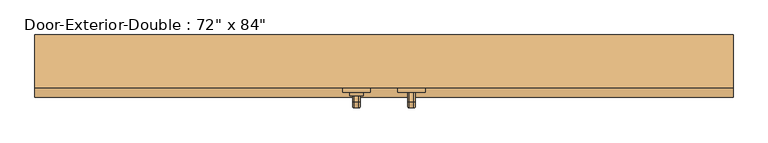
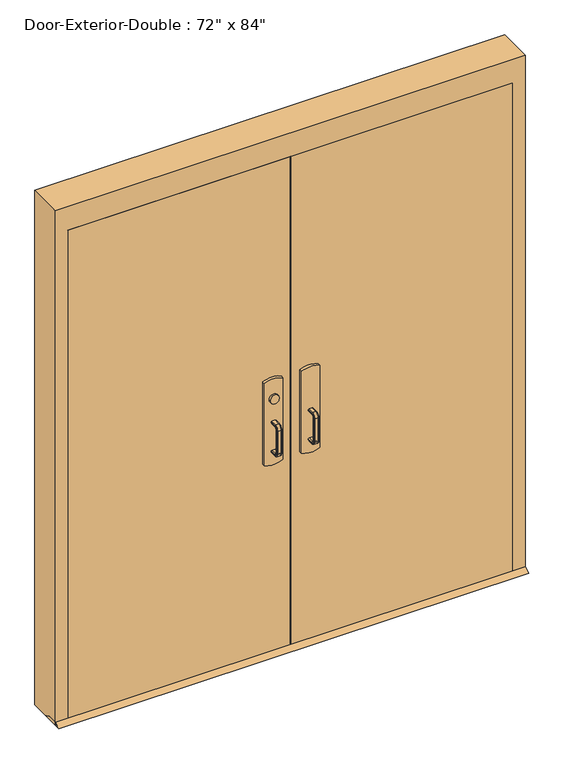
"""IFC4 building model written with IfcOpenShell, lengths in millimetres: door geometry."""

from ifc_helpers import new_model, si_unit, point, frame, frame_2d, origin, place, context, project, spatial, polyline, circle_curve, ellipse_curve, trimmed, segment, composite_curve, outline, extrude, faceted_brep, source, transform, mapped, element, save
from ifc_brep_helpers import plane_surface, cylinder_surface, revolved_surface, advanced_brep


def door_02051829(model_context):
    return source(origin(), model_context, "Body", "SolidModel", [
        extrude(outline(polyline([(-575.7333333, 0.0), (-76.2, 0.0), (-76.2, -6.35), (-575.7333333, -6.35), (-575.7333333, 0.0)])), frame((0.0, 0.0, 990.6), z_axis=(0.0, 0.0, 1.0), x_axis=(1.0, 0.0, 0.0)), (0.0, 0.0, 1.0), 50.8),
        advanced_brep(
        [(-12.7, -6.35, 1041.4), (-12.7, -6.35, 990.6), (-76.2, -6.35, 990.6), (-825.5, -6.35, 990.6), (-825.5, -6.35, 1041.4), (-76.2, -6.35, 1041.4), (-825.5, -38.1, 1041.4), (-825.5, -38.1, 990.6), (-76.2, -38.1, 990.6), (-76.2, -38.1, 927.1), (-57.15, -38.1, 908.05), (-31.75, -38.1, 908.05), (-12.7, -38.1, 927.1), (-12.7, -38.1, 1104.9), (-31.75, -38.1, 1123.95), (-57.15, -38.1, 1123.95), (-76.2, -38.1, 1104.9), (-76.2, -38.1, 1041.4), (-76.2, -9.5252467, 1041.4), (-12.7, -9.5252467, 1041.4), (-12.7, -14.5354269, 1104.9), (-12.7, -14.5354269, 927.1), (-12.7, -9.5252467, 990.6), (-76.2, -9.5252467, 990.6), (-76.2, -14.5354269, 1104.9), (-76.2, -14.5354269, 927.1), (-31.75, -16.038481, 1123.95), (-57.15, -16.038481, 1123.95), (-57.15, -16.038481, 908.05), (-31.75, -16.038481, 908.05)],
        [
            (0, 1),
            (1, 2),
            (2, 3),
            (3, 4),
            (4, 5),
            (5, 0),
            (6, 7),
            (7, 8),
            (8, 9),
            (9, 10, circle_curve(frame((-57.15, -38.1, 927.1), z_axis=(0.0, -1.0, 0.0), x_axis=(-1.0, 0.0, 0.0)), 19.05)),
            (10, 11),
            (11, 12, circle_curve(frame((-31.75, -38.1, 927.1), z_axis=(0.0, -1.0, 0.0), x_axis=(-1.0, 0.0, 0.0)), 19.05)),
            (12, 13),
            (13, 14, circle_curve(frame((-31.75, -38.1, 1104.9), z_axis=(0.0, -1.0, 0.0), x_axis=(-1.0, 0.0, 0.0)), 19.05)),
            (14, 15),
            (15, 16, circle_curve(frame((-57.15, -38.1, 1104.9), z_axis=(0.0, -1.0, 0.0), x_axis=(-1.0, 0.0, 0.0)), 19.05)),
            (16, 17),
            (17, 6),
            (4, 6),
            (17, 18),
            (18, 19),
            (19, 0),
            (19, 20),
            (20, 13),
            (12, 21),
            (21, 22),
            (22, 1),
            (7, 3),
            (22, 23),
            (23, 8),
            (16, 24),
            (24, 18),
            (23, 25),
            (25, 9),
            (14, 26),
            (26, 27),
            (27, 15),
            (10, 28),
            (28, 29),
            (29, 11),
            (25, 28, ellipse_curve(frame((-57.15, -14.5354269, 927.1), z_axis=(0.0, -0.9969018152893365, 0.07865602756830282), x_axis=(0.0, 0.07865602756830208, 0.9969018152893365)), 19.1092038, 19.05)),
            (27, 24, ellipse_curve(frame((-57.15, -14.5354269, 1104.9), z_axis=(0.0, -0.9969018152893376, -0.07865602756828934), x_axis=(0.0, 0.078656027568288, -0.9969018152893377)), 19.1092038, 19.05)),
            (20, 26, ellipse_curve(frame((-31.75, -14.5354269, 1104.9), z_axis=(0.0, -0.9969018152893376, -0.07865602756828934), x_axis=(0.0, 0.078656027568288, -0.9969018152893377)), 19.1092038, 19.05)),
            (29, 21, ellipse_curve(frame((-31.75, -14.5354269, 927.1), z_axis=(0.0, -0.9969018152893365, 0.07865602756830282), x_axis=(0.0, 0.07865602756830208, 0.9969018152893365)), 19.1092038, 19.05)),
        ],
        [
            plane_surface(frame((-12.7, -6.35, 1041.4), z_axis=(0.0, 1.0, 0.0), x_axis=(1.0, 0.0, 0.0))),
            plane_surface(frame((-12.7, -38.1, 1041.4), z_axis=(0.0, -1.0, 0.0), x_axis=(-1.0, 0.0, 0.0))),
            plane_surface(frame((-825.5, -6.35, 1041.4), z_axis=(0.0, 0.0, 1.0), x_axis=(0.0, -1.0, 0.0))),
            plane_surface(frame((-12.7, -6.35, 1041.4), z_axis=(1.0, 0.0, 0.0), x_axis=(0.0, -1.0, 0.0))),
            plane_surface(frame((-12.7, -6.35, 990.6), z_axis=(0.0, 0.0, -1.0), x_axis=(0.0, -1.0, 0.0))),
            plane_surface(frame((-825.5, -6.35, 990.6), z_axis=(-1.0, 0.0, 0.0), x_axis=(0.0, -1.0, 0.0))),
            plane_surface(frame((-76.2, -9.5252467, 927.1), z_axis=(-1.0, 0.0, 0.0), x_axis=(0.0, -1.0, 0.0))),
            plane_surface(frame((-57.15, -9.5252467, 1123.95), z_axis=(0.0, 0.0, 1.0), x_axis=(0.0, -1.0, 0.0))),
            plane_surface(frame((-31.75, -9.5252467, 908.05), z_axis=(0.0, 0.0, -1.0), x_axis=(0.0, -1.0, 0.0))),
            cylinder_surface(frame((-57.15, -38.1, 927.1), z_axis=(0.0, 1.0, 0.0), x_axis=(-1.0, 0.0, 0.0)), 19.05),
            cylinder_surface(frame((-57.15, -38.1, 1104.9), z_axis=(0.0, 1.0, 0.0), x_axis=(-1.0, 0.0, 0.0)), 19.05),
            cylinder_surface(frame((-31.75, -38.1, 1104.9), z_axis=(0.0, 1.0, 0.0), x_axis=(-1.0, 0.0, 0.0)), 19.05),
            cylinder_surface(frame((-31.75, -38.1, 927.1), z_axis=(0.0, 1.0, 0.0), x_axis=(-1.0, 0.0, 0.0)), 19.05),
            plane_surface(frame((-76.2, -9.5252467, 1041.4), z_axis=(0.0, 0.9969018152893376, 0.07865602756828934), x_axis=(1.0, 0.0, 0.0))),
            plane_surface(frame((-76.2, -16.038481, 908.05), z_axis=(0.0, 0.9969018152893365, -0.07865602756830282), x_axis=(1.0, 0.0, 0.0))),
        ],
        [
            (0, [[1, 2, 3, 4, 5, 6]]),
            (1, [[7, 8, 9, 10, 11, 12, 13, 14, 15, 16, 17, 18]]),
            (2, [[19, -18, 20, 21, 22, -6, -5]]),
            (3, [[-1, -22, 23, 24, -13, 25, 26, 27]]),
            (4, [[28, -3, -2, -27, 29, 30, -8]]),
            (5, [[-4, -28, -7, -19]]),
            (6, [[-17, 31, 32, -20]]),
            (6, [[-9, -30, 33, 34]]),
            (7, [[-15, 35, 36, 37]]),
            (8, [[-11, 38, 39, 40]]),
            (9, [[-10, -34, 41, -38]]),
            (10, [[-16, -37, 42, -31]]),
            (11, [[-14, -24, 43, -35]]),
            (12, [[-12, -40, 44, -25]]),
            (13, [[-21, -32, -42, -36, -43, -23]]),
            (14, [[-26, -44, -39, -41, -33, -29]]),
        ],
    ),
        extrude(outline(polyline([(-82.55, 12.7), (-38.1, 12.7), (-12.7, 0.0), (-107.95, 0.0), (-82.55, 12.7)])), frame((-965.2, 0.0, 0.0), z_axis=(1.0, 0.0, 0.0), x_axis=(0.0, 1.0, 0.0)), (0.0, 0.0, 1.0), 1930.4),
        extrude(outline(polyline([(575.7333333, 0.0), (575.7333333, -6.35), (76.2, -6.35), (76.2, 0.0), (575.7333333, 0.0)])), frame((0.0, 0.0, 990.6), z_axis=(0.0, 0.0, 1.0), x_axis=(1.0, 0.0, 0.0)), (0.0, 0.0, 1.0), 50.8),
        advanced_brep(
        [(12.7, -6.35, 1041.4), (76.2, -6.35, 1041.4), (825.5, -6.35, 1041.4), (825.5, -6.35, 990.6), (76.2, -6.35, 990.6), (12.7, -6.35, 990.6), (825.5, -38.1, 1041.4), (76.2, -38.1, 1041.4), (76.2, -38.1, 1104.9), (57.15, -38.1, 1123.95), (31.75, -38.1, 1123.95), (12.7, -38.1, 1104.9), (12.7, -38.1, 927.1), (31.75, -38.1, 908.05), (57.15, -38.1, 908.05), (76.2, -38.1, 927.1), (76.2, -38.1, 990.6), (825.5, -38.1, 990.6), (12.7, -9.5252467, 1041.4), (76.2, -9.5252467, 1041.4), (12.7, -9.5252467, 990.6), (12.7, -14.5354269, 927.1), (12.7, -14.5354269, 1104.9), (76.2, -9.5252467, 990.6), (76.2, -14.5354269, 1104.9), (76.2, -14.5354269, 927.1), (57.15, -16.038481, 1123.95), (31.75, -16.038481, 1123.95), (31.75, -16.038481, 908.05), (57.15, -16.038481, 908.05)],
        [
            (0, 1),
            (1, 2),
            (2, 3),
            (3, 4),
            (4, 5),
            (5, 0),
            (6, 7),
            (7, 8),
            (8, 9, circle_curve(frame((57.15, -38.1, 1104.9), z_axis=(0.0, -1.0, 0.0), x_axis=(1.0, 0.0, 0.0)), 19.05)),
            (9, 10),
            (10, 11, circle_curve(frame((31.75, -38.1, 1104.9), z_axis=(0.0, -1.0, 0.0), x_axis=(1.0, 0.0, 0.0)), 19.05)),
            (11, 12),
            (12, 13, circle_curve(frame((31.75, -38.1, 927.1), z_axis=(0.0, -1.0, 0.0), x_axis=(1.0, 0.0, 0.0)), 19.05)),
            (13, 14),
            (14, 15, circle_curve(frame((57.15, -38.1, 927.1), z_axis=(0.0, -1.0, 0.0), x_axis=(1.0, 0.0, 0.0)), 19.05)),
            (15, 16),
            (16, 17),
            (17, 6),
            (0, 18),
            (18, 19),
            (19, 7),
            (6, 2),
            (5, 20),
            (20, 21),
            (21, 12),
            (11, 22),
            (22, 18),
            (16, 23),
            (23, 20),
            (3, 17),
            (19, 24),
            (24, 8),
            (15, 25),
            (25, 23),
            (9, 26),
            (26, 27),
            (27, 10),
            (13, 28),
            (28, 29),
            (29, 14),
            (29, 25, ellipse_curve(frame((57.15, -14.5354269, 927.1), z_axis=(0.0, -0.9969018152893365, 0.07865602756830282), x_axis=(0.0, 0.07865602756830208, 0.9969018152893365)), 19.1092038, 19.05)),
            (24, 26, ellipse_curve(frame((57.15, -14.5354269, 1104.9), z_axis=(0.0, -0.9969018152893376, -0.07865602756828934), x_axis=(0.0, 0.078656027568288, -0.9969018152893377)), 19.1092038, 19.05)),
            (27, 22, ellipse_curve(frame((31.75, -14.5354269, 1104.9), z_axis=(0.0, -0.9969018152893376, -0.07865602756828934), x_axis=(0.0, 0.078656027568288, -0.9969018152893377)), 19.1092038, 19.05)),
            (21, 28, ellipse_curve(frame((31.75, -14.5354269, 927.1), z_axis=(0.0, -0.9969018152893365, 0.07865602756830282), x_axis=(0.0, 0.07865602756830208, 0.9969018152893365)), 19.1092038, 19.05)),
        ],
        [
            plane_surface(frame((12.7, -6.35, 1041.4), z_axis=(0.0, 1.0, 0.0), x_axis=(-1.0, 0.0, 0.0))),
            plane_surface(frame((12.7, -38.1, 1041.4), z_axis=(0.0, -1.0, 0.0), x_axis=(1.0, 0.0, 0.0))),
            plane_surface(frame((825.5, -6.35, 1041.4), z_axis=(0.0, 0.0, 1.0), x_axis=(0.0, -1.0, 0.0))),
            plane_surface(frame((12.7, -6.35, 1041.4), z_axis=(-1.0, 0.0, 0.0), x_axis=(0.0, -1.0, 0.0))),
            plane_surface(frame((12.7, -6.35, 990.6), z_axis=(0.0, 0.0, -1.0), x_axis=(0.0, -1.0, 0.0))),
            plane_surface(frame((825.5, -6.35, 990.6), z_axis=(1.0, 0.0, 0.0), x_axis=(0.0, -1.0, 0.0))),
            plane_surface(frame((76.2, -9.5252467, 927.1), z_axis=(1.0, 0.0, 0.0), x_axis=(0.0, -1.0, 0.0))),
            plane_surface(frame((57.15, -9.5252467, 1123.95), z_axis=(0.0, 0.0, 1.0), x_axis=(0.0, -1.0, 0.0))),
            plane_surface(frame((31.75, -9.5252467, 908.05), z_axis=(0.0, 0.0, -1.0), x_axis=(0.0, -1.0, 0.0))),
            cylinder_surface(frame((57.15, -38.1, 927.1), z_axis=(0.0, 1.0, 0.0), x_axis=(1.0, 0.0, 0.0)), 19.05),
            cylinder_surface(frame((57.15, -38.1, 1104.9), z_axis=(0.0, 1.0, 0.0), x_axis=(1.0, 0.0, 0.0)), 19.05),
            cylinder_surface(frame((31.75, -38.1, 1104.9), z_axis=(0.0, 1.0, 0.0), x_axis=(1.0, 0.0, 0.0)), 19.05),
            cylinder_surface(frame((31.75, -38.1, 927.1), z_axis=(0.0, 1.0, 0.0), x_axis=(1.0, 0.0, 0.0)), 19.05),
            plane_surface(frame((76.2, -9.5252467, 1041.4), z_axis=(0.0, 0.9969018152893376, 0.07865602756828934), x_axis=(-1.0, 0.0, 0.0))),
            plane_surface(frame((76.2, -16.038481, 908.05), z_axis=(0.0, 0.9969018152893365, -0.07865602756830282), x_axis=(-1.0, 0.0, 0.0))),
        ],
        [
            (0, [[1, 2, 3, 4, 5, 6]]),
            (1, [[7, 8, 9, 10, 11, 12, 13, 14, 15, 16, 17, 18]]),
            (2, [[-2, -1, 19, 20, 21, -7, 22]]),
            (3, [[23, 24, 25, -12, 26, 27, -19, -6]]),
            (4, [[-17, 28, 29, -23, -5, -4, 30]]),
            (5, [[-22, -18, -30, -3]]),
            (6, [[-21, 31, 32, -8]]),
            (6, [[33, 34, -28, -16]]),
            (7, [[35, 36, 37, -10]]),
            (8, [[38, 39, 40, -14]]),
            (9, [[-40, 41, -33, -15]]),
            (10, [[-32, 42, -35, -9]]),
            (11, [[-37, 43, -26, -11]]),
            (12, [[-25, 44, -38, -13]]),
            (13, [[-27, -43, -36, -42, -31, -20]]),
            (14, [[-29, -34, -41, -39, -44, -24]]),
        ],
    ),
        advanced_brep(
        [(66.2, -95.25, 1017.190625), (69.771875, -95.25, 1020.7625), (82.628125, -95.25, 1020.7625), (86.2, -95.25, 1017.190625), (86.2, -95.25, 1014.8090406), (82.6284594, -95.25, 1011.2375), (69.771875, -95.25, 1011.2375), (66.2, -95.25, 1014.809375), (66.2, -95.25, 887.809375), (66.2, -95.25, 890.190625), (69.771875, -95.25, 893.7625), (82.6284594, -95.25, 893.7625), (86.2, -95.25, 890.1909594), (86.2, -95.25, 887.809375), (82.628125, -95.25, 884.2375), (69.771875, -95.25, 884.2375), (66.2, -120.65, 1014.809375), (66.2, -132.159375, 1003.3), (66.2, -132.159375, 901.7), (66.2, -120.65, 890.190625), (66.2, -120.65, 887.809375), (66.2, -134.540625, 901.7), (66.2, -134.540625, 1003.3), (66.2, -120.65, 1017.190625), (69.771875, -120.65, 1011.2375), (82.6284594, -120.65, 1011.2375), (86.2, -120.65, 1014.8090406), (86.2, -120.65, 1017.190625), (86.2, -134.540625, 1003.3), (86.2, -134.540625, 901.7), (86.2, -120.65, 887.809375), (86.2, -120.65, 890.1909594), (86.2, -132.1590406, 901.7), (86.2, -132.1590406, 1003.3), (82.628125, -120.65, 1020.7625), (69.771875, -120.65, 1020.7625), (69.771875, -128.5875, 1003.3), (82.6284594, -128.5875, 1003.3), (82.628125, -138.1125, 1003.3), (69.771875, -138.1125, 1003.3), (69.771875, -128.5875, 901.7), (82.6284594, -128.5875, 901.7), (82.628125, -138.1125, 901.7), (69.771875, -138.1125, 901.7), (69.771875, -120.65, 893.7625), (82.6284594, -120.65, 893.7625), (82.628125, -120.65, 884.2375), (69.771875, -120.65, 884.2375)],
        [
            (0, 1, circle_curve(frame((69.771875, -95.25, 1017.190625), z_axis=(0.0, 1.0, 0.0), x_axis=(0.0, 0.0, 1.0)), 3.571875)),
            (1, 2),
            (2, 3, circle_curve(frame((82.628125, -95.25, 1017.190625), z_axis=(0.0, 1.0, 0.0), x_axis=(0.0, 0.0, 1.0)), 3.571875)),
            (3, 4),
            (4, 5, circle_curve(frame((82.6284594, -95.25, 1014.8090406), z_axis=(0.0, 1.0, 0.0), x_axis=(0.0, 0.0, 1.0)), 3.5715406)),
            (5, 6),
            (6, 7, circle_curve(frame((69.771875, -95.25, 1014.809375), z_axis=(0.0, 1.0, 0.0), x_axis=(0.0, 0.0, 1.0)), 3.571875)),
            (7, 0),
            (8, 9),
            (9, 10, circle_curve(frame((69.771875, -95.25, 890.190625), z_axis=(0.0, 1.0, 0.0), x_axis=(0.0, 0.0, -1.0)), 3.571875)),
            (10, 11),
            (11, 12, circle_curve(frame((82.6284594, -95.25, 890.1909594), z_axis=(0.0, 1.0, 0.0), x_axis=(0.0, 0.0, -1.0)), 3.5715406)),
            (12, 13),
            (13, 14, circle_curve(frame((82.628125, -95.25, 887.809375), z_axis=(0.0, 1.0, 0.0), x_axis=(0.0, 0.0, -1.0)), 3.571875)),
            (14, 15),
            (15, 8, circle_curve(frame((69.771875, -95.25, 887.809375), z_axis=(0.0, 1.0, 0.0), x_axis=(0.0, 0.0, -1.0)), 3.571875)),
            (7, 16),
            (16, 17, circle_curve(frame((66.2, -120.65, 1003.3), z_axis=(1.0, 0.0, 0.0), x_axis=(0.0, 0.0, 1.0)), 11.509375)),
            (17, 18),
            (18, 19, circle_curve(frame((66.2, -120.65, 901.7), z_axis=(1.0, 0.0, 0.0), x_axis=(0.0, -1.0, 0.0)), 11.509375)),
            (19, 9),
            (8, 20),
            (20, 21, circle_curve(frame((66.2, -120.65, 901.7), z_axis=(-1.0, 0.0, 0.0), x_axis=(0.0, -1.0, 0.0)), 13.890625)),
            (21, 22),
            (22, 23, circle_curve(frame((66.2, -120.65, 1003.3), z_axis=(-1.0, 0.0, 0.0), x_axis=(0.0, 0.0, 1.0)), 13.890625)),
            (23, 0),
            (6, 24),
            (24, 16, circle_curve(frame((69.771875, -120.65, 1014.809375), z_axis=(0.0, 1.0, 0.0), x_axis=(0.0, 0.0, 1.0)), 3.571875)),
            (5, 25),
            (25, 24),
            (4, 26),
            (26, 25, circle_curve(frame((82.6284594, -120.65, 1014.8090406), z_axis=(0.0, 1.0, 0.0), x_axis=(0.0, 0.0, 1.0)), 3.5715406)),
            (3, 27),
            (27, 28, circle_curve(frame((86.2, -120.65, 1003.3), z_axis=(1.0, 0.0, 0.0), x_axis=(0.0, 0.0, 1.0)), 13.890625)),
            (28, 29),
            (29, 30, circle_curve(frame((86.2, -120.65, 901.7), z_axis=(1.0, 0.0, 0.0), x_axis=(0.0, -1.0, 0.0)), 13.890625)),
            (30, 13),
            (12, 31),
            (31, 32, circle_curve(frame((86.2, -120.65, 901.7), z_axis=(-1.0, 0.0, 0.0), x_axis=(0.0, -1.0, 0.0)), 11.5090406)),
            (32, 33),
            (33, 26, circle_curve(frame((86.2, -120.65, 1003.3), z_axis=(-1.0, 0.0, 0.0), x_axis=(0.0, 0.0, 1.0)), 11.5090406)),
            (2, 34),
            (34, 27, circle_curve(frame((82.628125, -120.65, 1017.190625), z_axis=(0.0, 1.0, 0.0), x_axis=(0.0, 0.0, 1.0)), 3.571875)),
            (1, 35),
            (35, 34),
            (23, 35, circle_curve(frame((69.771875, -120.65, 1017.190625), z_axis=(0.0, 1.0, 0.0), x_axis=(0.0, 0.0, 1.0)), 3.571875)),
            (36, 17, circle_curve(frame((69.771875, -132.159375, 1003.3), z_axis=(0.0, 0.0, 1.0), x_axis=(0.0, -1.0, 0.0)), 3.571875)),
            (24, 36, circle_curve(frame((69.771875, -120.65, 1003.3), z_axis=(1.0, 0.0, 0.0), x_axis=(0.0, 0.0, 1.0)), 7.9375)),
            (37, 36),
            (25, 37, circle_curve(frame((82.6284594, -120.65, 1003.3), z_axis=(1.0, 0.0, 0.0), x_axis=(0.0, 0.0, 1.0)), 7.9375)),
            (33, 37, circle_curve(frame((82.6284594, -132.1590406, 1003.3), z_axis=(0.0, 0.0, 1.0), x_axis=(0.0, -1.0, 0.0)), 3.5715406)),
            (38, 28, circle_curve(frame((82.628125, -134.540625, 1003.3), z_axis=(0.0, 0.0, 1.0), x_axis=(0.0, -1.0, 0.0)), 3.571875)),
            (34, 38, circle_curve(frame((82.628125, -120.65, 1003.3), z_axis=(1.0, 0.0, 0.0), x_axis=(0.0, 0.0, 1.0)), 17.4625)),
            (39, 38),
            (35, 39, circle_curve(frame((69.771875, -120.65, 1003.3), z_axis=(1.0, 0.0, 0.0), x_axis=(0.0, 0.0, 1.0)), 17.4625)),
            (22, 39, circle_curve(frame((69.771875, -134.540625, 1003.3), z_axis=(0.0, 0.0, 1.0), x_axis=(0.0, -1.0, 0.0)), 3.571875)),
            (36, 40),
            (40, 18, circle_curve(frame((69.771875, -132.159375, 901.7), z_axis=(0.0, 0.0, 1.0), x_axis=(0.0, -1.0, 0.0)), 3.571875)),
            (37, 41),
            (41, 40),
            (32, 41, circle_curve(frame((82.6284594, -132.1590406, 901.7), z_axis=(0.0, 0.0, 1.0), x_axis=(0.0, -1.0, 0.0)), 3.5715406)),
            (38, 42),
            (42, 29, circle_curve(frame((82.628125, -134.540625, 901.7), z_axis=(0.0, 0.0, 1.0), x_axis=(0.0, -1.0, 0.0)), 3.571875)),
            (39, 43),
            (43, 42),
            (21, 43, circle_curve(frame((69.771875, -134.540625, 901.7), z_axis=(0.0, 0.0, 1.0), x_axis=(0.0, -1.0, 0.0)), 3.571875)),
            (44, 19, circle_curve(frame((69.771875, -120.65, 890.190625), z_axis=(0.0, -1.0, 0.0), x_axis=(0.0, 0.0, -1.0)), 3.571875)),
            (40, 44, circle_curve(frame((69.771875, -120.65, 901.7), z_axis=(1.0, 0.0, 0.0), x_axis=(0.0, -1.0, 0.0)), 7.9375)),
            (45, 44),
            (41, 45, circle_curve(frame((82.6284594, -120.65, 901.7), z_axis=(1.0, 0.0, 0.0), x_axis=(0.0, -1.0, 0.0)), 7.9375)),
            (31, 45, circle_curve(frame((82.6284594, -120.65, 890.1909594), z_axis=(0.0, -1.0, 0.0), x_axis=(0.0, 0.0, -1.0)), 3.5715406)),
            (46, 30, circle_curve(frame((82.628125, -120.65, 887.809375), z_axis=(0.0, -1.0, 0.0), x_axis=(0.0, 0.0, -1.0)), 3.571875)),
            (42, 46, circle_curve(frame((82.628125, -120.65, 901.7), z_axis=(1.0, 0.0, 0.0), x_axis=(0.0, -1.0, 0.0)), 17.4625)),
            (47, 46),
            (43, 47, circle_curve(frame((69.771875, -120.65, 901.7), z_axis=(1.0, 0.0, 0.0), x_axis=(0.0, -1.0, 0.0)), 17.4625)),
            (20, 47, circle_curve(frame((69.771875, -120.65, 887.809375), z_axis=(0.0, -1.0, 0.0), x_axis=(0.0, 0.0, -1.0)), 3.571875)),
            (44, 10),
            (45, 11),
            (46, 14),
            (47, 15),
        ],
        [
            plane_surface(frame((76.2, -95.25, 1016.0), z_axis=(0.0, 1.0, 0.0), x_axis=(1.0, 0.0, 0.0))),
            plane_surface(frame((76.2, -95.25, 889.0), z_axis=(0.0, 1.0, 0.0), x_axis=(1.0, 0.0, 0.0))),
            plane_surface(frame((66.2, -95.25, 1017.190625), z_axis=(-1.0, 0.0, 0.0), x_axis=(0.0, -1.0, 0.0))),
            cylinder_surface(frame((69.771875, -95.25, 1014.809375), z_axis=(0.0, 1.0, 0.0), x_axis=(0.0, 0.0, 1.0)), 3.571875),
            plane_surface(frame((69.771875, -95.25, 1011.2375), z_axis=(0.0, 0.0, -1.0), x_axis=(0.0, -1.0, 0.0))),
            cylinder_surface(frame((82.6284594, -95.25, 1014.8090406), z_axis=(0.0, 1.0, 0.0), x_axis=(0.0, 0.0, 1.0)), 3.5715406),
            plane_surface(frame((86.2, -95.25, 1014.8090406), z_axis=(1.0, 0.0, 0.0), x_axis=(0.0, -1.0, 0.0))),
            cylinder_surface(frame((82.628125, -95.25, 1017.190625), z_axis=(0.0, 1.0, 0.0), x_axis=(0.0, 0.0, 1.0)), 3.571875),
            plane_surface(frame((82.628125, -95.25, 1020.7625), z_axis=(0.0, 0.0, 1.0), x_axis=(0.0, -1.0, 0.0))),
            cylinder_surface(frame((69.771875, -95.25, 1017.190625), z_axis=(0.0, 1.0, 0.0), x_axis=(0.0, 0.0, 1.0)), 3.571875),
            revolved_surface(trimmed(ellipse_curve(frame((69.771875, -120.65, 1014.809375), z_axis=(0.0, -1.0, 0.0), x_axis=(0.0, 0.0, 1.0)), 3.571875, 3.571875), [point((66.2, -120.65, 1014.809375))], [point((69.771875, -120.65, 1011.2375))], True, "CARTESIAN"), (76.2, -120.65, 1003.3), (-1.0, 0.0, 0.0)),
            revolved_surface(polyline([(69.771875, -120.65, 1011.2375), (82.6284594, -120.65, 1011.2375)]), (76.2, -120.65, 1003.3), (-1.0, 0.0, 0.0)),
            revolved_surface(trimmed(ellipse_curve(frame((82.6284594, -120.65, 1014.8090406), z_axis=(0.0, -1.0, 0.0), x_axis=(0.0, 0.0, 1.0)), 3.5715406, 3.5715406), [point((82.6284594, -120.65, 1011.2375))], [point((86.2, -120.65, 1014.8090406))], True, "CARTESIAN"), (76.2, -120.65, 1003.3), (-1.0, 0.0, 0.0)),
            revolved_surface(trimmed(ellipse_curve(frame((82.628125, -120.65, 1017.190625), z_axis=(0.0, -1.0, 0.0), x_axis=(0.0, 0.0, 1.0)), 3.571875, 3.571875), [point((86.2, -120.65, 1017.190625))], [point((82.628125, -120.65, 1020.7625))], True, "CARTESIAN"), (76.2, -120.65, 1003.3), (-1.0, 0.0, 0.0)),
            cylinder_surface(frame((76.2, -120.65, 1003.3), z_axis=(-1.0, 0.0, 0.0), x_axis=(0.0, 0.0, 1.0)), 17.4625),
            revolved_surface(trimmed(ellipse_curve(frame((69.771875, -120.65, 1017.190625), z_axis=(0.0, -1.0, 0.0), x_axis=(0.0, 0.0, 1.0)), 3.571875, 3.571875), [point((69.771875, -120.65, 1020.7625))], [point((66.2, -120.65, 1017.190625))], True, "CARTESIAN"), (76.2, -120.65, 1003.3), (-1.0, 0.0, 0.0)),
            cylinder_surface(frame((69.771875, -132.159375, 1003.3), z_axis=(0.0, 0.0, 1.0), x_axis=(0.0, -1.0, 0.0)), 3.571875),
            plane_surface(frame((69.771875, -128.5875, 1003.3), z_axis=(0.0, 1.0, 0.0), x_axis=(0.0, 0.0, -1.0))),
            cylinder_surface(frame((82.6284594, -132.1590406, 1003.3), z_axis=(0.0, 0.0, 1.0), x_axis=(0.0, -1.0, 0.0)), 3.5715406),
            cylinder_surface(frame((82.628125, -134.540625, 1003.3), z_axis=(0.0, 0.0, 1.0), x_axis=(0.0, -1.0, 0.0)), 3.571875),
            plane_surface(frame((82.628125, -138.1125, 1003.3), z_axis=(0.0, -1.0, 0.0), x_axis=(0.0, 0.0, -1.0))),
            cylinder_surface(frame((69.771875, -134.540625, 1003.3), z_axis=(0.0, 0.0, 1.0), x_axis=(0.0, -1.0, 0.0)), 3.571875),
            revolved_surface(trimmed(ellipse_curve(frame((69.771875, -132.159375, 901.7), z_axis=(0.0, 0.0, -1.0), x_axis=(0.0, -1.0, 0.0)), 3.571875, 3.571875), [point((66.2, -132.159375, 901.7))], [point((69.771875, -128.5875, 901.7))], True, "CARTESIAN"), (76.2, -120.65, 901.7), (-1.0, 0.0, 0.0)),
            revolved_surface(polyline([(69.771875, -128.5875, 901.7), (82.6284594, -128.5875, 901.7)]), (76.2, -120.65, 901.7), (-1.0, 0.0, 0.0)),
            revolved_surface(trimmed(ellipse_curve(frame((82.6284594, -132.1590406, 901.7), z_axis=(0.0, 0.0, -1.0), x_axis=(0.0, -1.0, 0.0)), 3.5715406, 3.5715406), [point((82.6284594, -128.5875, 901.7))], [point((86.2, -132.1590406, 901.7))], True, "CARTESIAN"), (76.2, -120.65, 901.7), (-1.0, 0.0, 0.0)),
            revolved_surface(trimmed(ellipse_curve(frame((82.628125, -134.540625, 901.7), z_axis=(0.0, 0.0, -1.0), x_axis=(0.0, -1.0, 0.0)), 3.571875, 3.571875), [point((86.2, -134.540625, 901.7))], [point((82.628125, -138.1125, 901.7))], True, "CARTESIAN"), (76.2, -120.65, 901.7), (-1.0, 0.0, 0.0)),
            cylinder_surface(frame((76.2, -120.65, 901.7), z_axis=(-1.0, 0.0, 0.0), x_axis=(0.0, -1.0, 0.0)), 17.4625),
            revolved_surface(trimmed(ellipse_curve(frame((69.771875, -134.540625, 901.7), z_axis=(0.0, 0.0, -1.0), x_axis=(0.0, -1.0, 0.0)), 3.571875, 3.571875), [point((69.771875, -138.1125, 901.7))], [point((66.2, -134.540625, 901.7))], True, "CARTESIAN"), (76.2, -120.65, 901.7), (-1.0, 0.0, 0.0)),
            cylinder_surface(frame((69.771875, -120.65, 890.190625), z_axis=(0.0, -1.0, 0.0), x_axis=(0.0, 0.0, -1.0)), 3.571875),
            plane_surface(frame((69.771875, -120.65, 893.7625), z_axis=(0.0, 0.0, 1.0), x_axis=(0.0, 1.0, 0.0))),
            cylinder_surface(frame((82.6284594, -120.65, 890.1909594), z_axis=(0.0, -1.0, 0.0), x_axis=(0.0, 0.0, -1.0)), 3.5715406),
            cylinder_surface(frame((82.628125, -120.65, 887.809375), z_axis=(0.0, -1.0, 0.0), x_axis=(0.0, 0.0, -1.0)), 3.571875),
            plane_surface(frame((82.628125, -120.65, 884.2375), z_axis=(0.0, 0.0, -1.0), x_axis=(0.0, 1.0, 0.0))),
            cylinder_surface(frame((69.771875, -120.65, 887.809375), z_axis=(0.0, -1.0, 0.0), x_axis=(0.0, 0.0, -1.0)), 3.571875),
        ],
        [
            (0, [[1, 2, 3, 4, 5, 6, 7, 8]]),
            (1, [[9, 10, 11, 12, 13, 14, 15, 16]]),
            (2, [[17, 18, 19, 20, 21, -9, 22, 23, 24, 25, 26, -8]]),
            (3, [[27, 28, -17, -7]]),
            (4, [[29, 30, -27, -6]]),
            (5, [[31, 32, -29, -5]]),
            (6, [[33, 34, 35, 36, 37, -13, 38, 39, 40, 41, -31, -4]]),
            (7, [[42, 43, -33, -3]]),
            (8, [[44, 45, -42, -2]]),
            (9, [[-26, 46, -44, -1]]),
            (10, [[47, -18, -28, 48]]),
            (11, [[49, -48, -30, 50]]),
            (12, [[51, -50, -32, -41]]),
            (13, [[52, -34, -43, 53]]),
            (14, [[54, -53, -45, 55]]),
            (15, [[56, -55, -46, -25]]),
            (16, [[57, 58, -19, -47]]),
            (17, [[59, 60, -57, -49]]),
            (18, [[-40, 61, -59, -51]]),
            (19, [[62, 63, -35, -52]]),
            (20, [[64, 65, -62, -54]]),
            (21, [[-24, 66, -64, -56]]),
            (22, [[67, -20, -58, 68]]),
            (23, [[69, -68, -60, 70]]),
            (24, [[71, -70, -61, -39]]),
            (25, [[72, -36, -63, 73]]),
            (26, [[74, -73, -65, 75]]),
            (27, [[76, -75, -66, -23]]),
            (28, [[77, -10, -21, -67]]),
            (29, [[78, -11, -77, -69]]),
            (30, [[-38, -12, -78, -71]]),
            (31, [[79, -14, -37, -72]]),
            (32, [[80, -15, -79, -74]]),
            (33, [[-22, -16, -80, -76]]),
        ],
    ),
        extrude(outline(composite_curve([segment(trimmed(circle_curve(frame_2d((1113.0338574, 76.2)), 89.3016225), [point((1193.8, 114.3))], [point((1193.8, 38.1))], False, "CARTESIAN"), True, "CONTINUOUS"), segment(polyline([(1193.8, 38.1), (838.2, 38.1)]), True, "CONTINUOUS"), segment(trimmed(circle_curve(frame_2d((918.9661426, 76.2)), 89.3016225), [point((838.2, 38.1))], [point((838.2, 114.3))], False, "CARTESIAN"), True, "CONTINUOUS"), segment(polyline([(838.2, 114.3), (1193.8, 114.3)]), True, "CONTINUOUS")], self_intersect=False)), frame((0.0, -95.25, 0.0), z_axis=(0.0, 1.0, 0.0), x_axis=(0.0, 0.0, 1.0)), (0.0, 0.0, 1.0), 12.7),
        advanced_brep(
        [(-86.2, -95.25, 1017.190625), (-82.628125, -95.25, 1020.7625), (-69.771875, -95.25, 1020.7625), (-66.2, -95.25, 1017.190625), (-66.2, -95.25, 1014.8090406), (-69.7715406, -95.25, 1011.2375), (-82.628125, -95.25, 1011.2375), (-86.2, -95.25, 1014.809375), (-86.2, -95.25, 887.809375), (-86.2, -95.25, 890.190625), (-82.628125, -95.25, 893.7625), (-69.7715406, -95.25, 893.7625), (-66.2, -95.25, 890.1909594), (-66.2, -95.25, 887.809375), (-69.771875, -95.25, 884.2375), (-82.628125, -95.25, 884.2375), (-86.2, -120.65, 1014.809375), (-86.2, -132.159375, 1003.3), (-86.2, -132.159375, 901.7), (-86.2, -120.65, 890.190625), (-86.2, -120.65, 887.809375), (-86.2, -134.540625, 901.7), (-86.2, -134.540625, 1003.3), (-86.2, -120.65, 1017.190625), (-82.628125, -120.65, 1011.2375), (-69.7715406, -120.65, 1011.2375), (-66.2, -120.65, 1014.8090406), (-66.2, -120.65, 1017.190625), (-66.2, -134.540625, 1003.3), (-66.2, -134.540625, 901.7), (-66.2, -120.65, 887.809375), (-66.2, -120.65, 890.1909594), (-66.2, -132.1590406, 901.7), (-66.2, -132.1590406, 1003.3), (-69.771875, -120.65, 1020.7625), (-82.628125, -120.65, 1020.7625), (-82.628125, -128.5875, 1003.3), (-69.7715406, -128.5875, 1003.3), (-69.771875, -138.1125, 1003.3), (-82.628125, -138.1125, 1003.3), (-82.628125, -128.5875, 901.7), (-69.7715406, -128.5875, 901.7), (-69.771875, -138.1125, 901.7), (-82.628125, -138.1125, 901.7), (-82.628125, -120.65, 893.7625), (-69.7715406, -120.65, 893.7625), (-69.771875, -120.65, 884.2375), (-82.628125, -120.65, 884.2375)],
        [
            (0, 1, circle_curve(frame((-82.628125, -95.25, 1017.190625), z_axis=(0.0, 1.0, 0.0), x_axis=(0.0, 0.0, 1.0)), 3.571875)),
            (1, 2),
            (2, 3, circle_curve(frame((-69.771875, -95.25, 1017.190625), z_axis=(0.0, 1.0, 0.0), x_axis=(0.0, 0.0, 1.0)), 3.571875)),
            (3, 4),
            (4, 5, circle_curve(frame((-69.7715406, -95.25, 1014.8090406), z_axis=(0.0, 1.0, 0.0), x_axis=(0.0, 0.0, 1.0)), 3.5715406)),
            (5, 6),
            (6, 7, circle_curve(frame((-82.628125, -95.25, 1014.809375), z_axis=(0.0, 1.0, 0.0), x_axis=(0.0, 0.0, 1.0)), 3.571875)),
            (7, 0),
            (8, 9),
            (9, 10, circle_curve(frame((-82.628125, -95.25, 890.190625), z_axis=(0.0, 1.0, 0.0), x_axis=(0.0, 0.0, -1.0)), 3.571875)),
            (10, 11),
            (11, 12, circle_curve(frame((-69.7715406, -95.25, 890.1909594), z_axis=(0.0, 1.0, 0.0), x_axis=(0.0, 0.0, -1.0)), 3.5715406)),
            (12, 13),
            (13, 14, circle_curve(frame((-69.771875, -95.25, 887.809375), z_axis=(0.0, 1.0, 0.0), x_axis=(0.0, 0.0, -1.0)), 3.571875)),
            (14, 15),
            (15, 8, circle_curve(frame((-82.628125, -95.25, 887.809375), z_axis=(0.0, 1.0, 0.0), x_axis=(0.0, 0.0, -1.0)), 3.571875)),
            (7, 16),
            (16, 17, circle_curve(frame((-86.2, -120.65, 1003.3), z_axis=(1.0, 0.0, 0.0), x_axis=(0.0, 0.0, 1.0)), 11.509375)),
            (17, 18),
            (18, 19, circle_curve(frame((-86.2, -120.65, 901.7), z_axis=(1.0, 0.0, 0.0), x_axis=(0.0, -1.0, 0.0)), 11.509375)),
            (19, 9),
            (8, 20),
            (20, 21, circle_curve(frame((-86.2, -120.65, 901.7), z_axis=(-1.0, 0.0, 0.0), x_axis=(0.0, -1.0, 0.0)), 13.890625)),
            (21, 22),
            (22, 23, circle_curve(frame((-86.2, -120.65, 1003.3), z_axis=(-1.0, 0.0, 0.0), x_axis=(0.0, 0.0, 1.0)), 13.890625)),
            (23, 0),
            (6, 24),
            (24, 16, circle_curve(frame((-82.628125, -120.65, 1014.809375), z_axis=(0.0, 1.0, 0.0), x_axis=(0.0, 0.0, 1.0)), 3.571875)),
            (5, 25),
            (25, 24),
            (4, 26),
            (26, 25, circle_curve(frame((-69.7715406, -120.65, 1014.8090406), z_axis=(0.0, 1.0, 0.0), x_axis=(0.0, 0.0, 1.0)), 3.5715406)),
            (3, 27),
            (27, 28, circle_curve(frame((-66.2, -120.65, 1003.3), z_axis=(1.0, 0.0, 0.0), x_axis=(0.0, 0.0, 1.0)), 13.890625)),
            (28, 29),
            (29, 30, circle_curve(frame((-66.2, -120.65, 901.7), z_axis=(1.0, 0.0, 0.0), x_axis=(0.0, -1.0, 0.0)), 13.890625)),
            (30, 13),
            (12, 31),
            (31, 32, circle_curve(frame((-66.2, -120.65, 901.7), z_axis=(-1.0, 0.0, 0.0), x_axis=(0.0, -1.0, 0.0)), 11.5090406)),
            (32, 33),
            (33, 26, circle_curve(frame((-66.2, -120.65, 1003.3), z_axis=(-1.0, 0.0, 0.0), x_axis=(0.0, 0.0, 1.0)), 11.5090406)),
            (2, 34),
            (34, 27, circle_curve(frame((-69.771875, -120.65, 1017.190625), z_axis=(0.0, 1.0, 0.0), x_axis=(0.0, 0.0, 1.0)), 3.571875)),
            (1, 35),
            (35, 34),
            (23, 35, circle_curve(frame((-82.628125, -120.65, 1017.190625), z_axis=(0.0, 1.0, 0.0), x_axis=(0.0, 0.0, 1.0)), 3.571875)),
            (36, 17, circle_curve(frame((-82.628125, -132.159375, 1003.3), z_axis=(0.0, 0.0, 1.0), x_axis=(0.0, -1.0, 0.0)), 3.571875)),
            (24, 36, circle_curve(frame((-82.628125, -120.65, 1003.3), z_axis=(1.0, 0.0, 0.0), x_axis=(0.0, 0.0, 1.0)), 7.9375)),
            (37, 36),
            (25, 37, circle_curve(frame((-69.7715406, -120.65, 1003.3), z_axis=(1.0, 0.0, 0.0), x_axis=(0.0, 0.0, 1.0)), 7.9375)),
            (33, 37, circle_curve(frame((-69.7715406, -132.1590406, 1003.3), z_axis=(0.0, 0.0, 1.0), x_axis=(0.0, -1.0, 0.0)), 3.5715406)),
            (38, 28, circle_curve(frame((-69.771875, -134.540625, 1003.3), z_axis=(0.0, 0.0, 1.0), x_axis=(0.0, -1.0, 0.0)), 3.571875)),
            (34, 38, circle_curve(frame((-69.771875, -120.65, 1003.3), z_axis=(1.0, 0.0, 0.0), x_axis=(0.0, 0.0, 1.0)), 17.4625)),
            (39, 38),
            (35, 39, circle_curve(frame((-82.628125, -120.65, 1003.3), z_axis=(1.0, 0.0, 0.0), x_axis=(0.0, 0.0, 1.0)), 17.4625)),
            (22, 39, circle_curve(frame((-82.628125, -134.540625, 1003.3), z_axis=(0.0, 0.0, 1.0), x_axis=(0.0, -1.0, 0.0)), 3.571875)),
            (36, 40),
            (40, 18, circle_curve(frame((-82.628125, -132.159375, 901.7), z_axis=(0.0, 0.0, 1.0), x_axis=(0.0, -1.0, 0.0)), 3.571875)),
            (37, 41),
            (41, 40),
            (32, 41, circle_curve(frame((-69.7715406, -132.1590406, 901.7), z_axis=(0.0, 0.0, 1.0), x_axis=(0.0, -1.0, 0.0)), 3.5715406)),
            (38, 42),
            (42, 29, circle_curve(frame((-69.771875, -134.540625, 901.7), z_axis=(0.0, 0.0, 1.0), x_axis=(0.0, -1.0, 0.0)), 3.571875)),
            (39, 43),
            (43, 42),
            (21, 43, circle_curve(frame((-82.628125, -134.540625, 901.7), z_axis=(0.0, 0.0, 1.0), x_axis=(0.0, -1.0, 0.0)), 3.571875)),
            (44, 19, circle_curve(frame((-82.628125, -120.65, 890.190625), z_axis=(0.0, -1.0, 0.0), x_axis=(0.0, 0.0, -1.0)), 3.571875)),
            (40, 44, circle_curve(frame((-82.628125, -120.65, 901.7), z_axis=(1.0, 0.0, 0.0), x_axis=(0.0, -1.0, 0.0)), 7.9375)),
            (45, 44),
            (41, 45, circle_curve(frame((-69.7715406, -120.65, 901.7), z_axis=(1.0, 0.0, 0.0), x_axis=(0.0, -1.0, 0.0)), 7.9375)),
            (31, 45, circle_curve(frame((-69.7715406, -120.65, 890.1909594), z_axis=(0.0, -1.0, 0.0), x_axis=(0.0, 0.0, -1.0)), 3.5715406)),
            (46, 30, circle_curve(frame((-69.771875, -120.65, 887.809375), z_axis=(0.0, -1.0, 0.0), x_axis=(0.0, 0.0, -1.0)), 3.571875)),
            (42, 46, circle_curve(frame((-69.771875, -120.65, 901.7), z_axis=(1.0, 0.0, 0.0), x_axis=(0.0, -1.0, 0.0)), 17.4625)),
            (47, 46),
            (43, 47, circle_curve(frame((-82.628125, -120.65, 901.7), z_axis=(1.0, 0.0, 0.0), x_axis=(0.0, -1.0, 0.0)), 17.4625)),
            (20, 47, circle_curve(frame((-82.628125, -120.65, 887.809375), z_axis=(0.0, -1.0, 0.0), x_axis=(0.0, 0.0, -1.0)), 3.571875)),
            (44, 10),
            (45, 11),
            (46, 14),
            (47, 15),
        ],
        [
            plane_surface(frame((-76.2, -95.25, 1016.0), z_axis=(0.0, 1.0, 0.0), x_axis=(1.0, 0.0, 0.0))),
            plane_surface(frame((-76.2, -95.25, 889.0), z_axis=(0.0, 1.0, 0.0), x_axis=(1.0, 0.0, 0.0))),
            plane_surface(frame((-86.2, -95.25, 1017.190625), z_axis=(-1.0, 0.0, 0.0), x_axis=(0.0, -1.0, 0.0))),
            cylinder_surface(frame((-82.628125, -95.25, 1014.809375), z_axis=(0.0, 1.0, 0.0), x_axis=(0.0, 0.0, 1.0)), 3.571875),
            plane_surface(frame((-82.628125, -95.25, 1011.2375), z_axis=(0.0, 0.0, -1.0), x_axis=(0.0, -1.0, 0.0))),
            cylinder_surface(frame((-69.7715406, -95.25, 1014.8090406), z_axis=(0.0, 1.0, 0.0), x_axis=(0.0, 0.0, 1.0)), 3.5715406),
            plane_surface(frame((-66.2, -95.25, 1014.8090406), z_axis=(1.0, 0.0, 0.0), x_axis=(0.0, -1.0, 0.0))),
            cylinder_surface(frame((-69.771875, -95.25, 1017.190625), z_axis=(0.0, 1.0, 0.0), x_axis=(0.0, 0.0, 1.0)), 3.571875),
            plane_surface(frame((-69.771875, -95.25, 1020.7625), z_axis=(0.0, 0.0, 1.0), x_axis=(0.0, -1.0, 0.0))),
            cylinder_surface(frame((-82.628125, -95.25, 1017.190625), z_axis=(0.0, 1.0, 0.0), x_axis=(0.0, 0.0, 1.0)), 3.571875),
            revolved_surface(trimmed(ellipse_curve(frame((-82.628125, -120.65, 1014.809375), z_axis=(0.0, -1.0, 0.0), x_axis=(0.0, 0.0, 1.0)), 3.571875, 3.571875), [point((-86.2, -120.65, 1014.809375))], [point((-82.628125, -120.65, 1011.2375))], True, "CARTESIAN"), (-76.2, -120.65, 1003.3), (-1.0, 0.0, 0.0)),
            revolved_surface(polyline([(-82.628125, -120.65, 1011.2375), (-69.7715406, -120.65, 1011.2375)]), (-76.2, -120.65, 1003.3), (-1.0, 0.0, 0.0)),
            revolved_surface(trimmed(ellipse_curve(frame((-69.7715406, -120.65, 1014.8090406), z_axis=(0.0, -1.0, 0.0), x_axis=(0.0, 0.0, 1.0)), 3.5715406, 3.5715406), [point((-69.7715406, -120.65, 1011.2375))], [point((-66.2, -120.65, 1014.8090406))], True, "CARTESIAN"), (-76.2, -120.65, 1003.3), (-1.0, 0.0, 0.0)),
            revolved_surface(trimmed(ellipse_curve(frame((-69.771875, -120.65, 1017.190625), z_axis=(0.0, -1.0, 0.0), x_axis=(0.0, 0.0, 1.0)), 3.571875, 3.571875), [point((-66.2, -120.65, 1017.190625))], [point((-69.771875, -120.65, 1020.7625))], True, "CARTESIAN"), (-76.2, -120.65, 1003.3), (-1.0, 0.0, 0.0)),
            cylinder_surface(frame((-76.2, -120.65, 1003.3), z_axis=(-1.0, 0.0, 0.0), x_axis=(0.0, 0.0, 1.0)), 17.4625),
            revolved_surface(trimmed(ellipse_curve(frame((-82.628125, -120.65, 1017.190625), z_axis=(0.0, -1.0, 0.0), x_axis=(0.0, 0.0, 1.0)), 3.571875, 3.571875), [point((-82.628125, -120.65, 1020.7625))], [point((-86.2, -120.65, 1017.190625))], True, "CARTESIAN"), (-76.2, -120.65, 1003.3), (-1.0, 0.0, 0.0)),
            cylinder_surface(frame((-82.628125, -132.159375, 1003.3), z_axis=(0.0, 0.0, 1.0), x_axis=(0.0, -1.0, 0.0)), 3.571875),
            plane_surface(frame((-82.628125, -128.5875, 1003.3), z_axis=(0.0, 1.0, 0.0), x_axis=(0.0, 0.0, -1.0))),
            cylinder_surface(frame((-69.7715406, -132.1590406, 1003.3), z_axis=(0.0, 0.0, 1.0), x_axis=(0.0, -1.0, 0.0)), 3.5715406),
            cylinder_surface(frame((-69.771875, -134.540625, 1003.3), z_axis=(0.0, 0.0, 1.0), x_axis=(0.0, -1.0, 0.0)), 3.571875),
            plane_surface(frame((-69.771875, -138.1125, 1003.3), z_axis=(0.0, -1.0, 0.0), x_axis=(0.0, 0.0, -1.0))),
            cylinder_surface(frame((-82.628125, -134.540625, 1003.3), z_axis=(0.0, 0.0, 1.0), x_axis=(0.0, -1.0, 0.0)), 3.571875),
            revolved_surface(trimmed(ellipse_curve(frame((-82.628125, -132.159375, 901.7), z_axis=(0.0, 0.0, -1.0), x_axis=(0.0, -1.0, 0.0)), 3.571875, 3.571875), [point((-86.2, -132.159375, 901.7))], [point((-82.628125, -128.5875, 901.7))], True, "CARTESIAN"), (-76.2, -120.65, 901.7), (-1.0, 0.0, 0.0)),
            revolved_surface(polyline([(-82.628125, -128.5875, 901.7), (-69.7715406, -128.5875, 901.7)]), (-76.2, -120.65, 901.7), (-1.0, 0.0, 0.0)),
            revolved_surface(trimmed(ellipse_curve(frame((-69.7715406, -132.1590406, 901.7), z_axis=(0.0, 0.0, -1.0), x_axis=(0.0, -1.0, 0.0)), 3.5715406, 3.5715406), [point((-69.7715406, -128.5875, 901.7))], [point((-66.2, -132.1590406, 901.7))], True, "CARTESIAN"), (-76.2, -120.65, 901.7), (-1.0, 0.0, 0.0)),
            revolved_surface(trimmed(ellipse_curve(frame((-69.771875, -134.540625, 901.7), z_axis=(0.0, 0.0, -1.0), x_axis=(0.0, -1.0, 0.0)), 3.571875, 3.571875), [point((-66.2, -134.540625, 901.7))], [point((-69.771875, -138.1125, 901.7))], True, "CARTESIAN"), (-76.2, -120.65, 901.7), (-1.0, 0.0, 0.0)),
            cylinder_surface(frame((-76.2, -120.65, 901.7), z_axis=(-1.0, 0.0, 0.0), x_axis=(0.0, -1.0, 0.0)), 17.4625),
            revolved_surface(trimmed(ellipse_curve(frame((-82.628125, -134.540625, 901.7), z_axis=(0.0, 0.0, -1.0), x_axis=(0.0, -1.0, 0.0)), 3.571875, 3.571875), [point((-82.628125, -138.1125, 901.7))], [point((-86.2, -134.540625, 901.7))], True, "CARTESIAN"), (-76.2, -120.65, 901.7), (-1.0, 0.0, 0.0)),
            cylinder_surface(frame((-82.628125, -120.65, 890.190625), z_axis=(0.0, -1.0, 0.0), x_axis=(0.0, 0.0, -1.0)), 3.571875),
            plane_surface(frame((-82.628125, -120.65, 893.7625), z_axis=(0.0, 0.0, 1.0), x_axis=(0.0, 1.0, 0.0))),
            cylinder_surface(frame((-69.7715406, -120.65, 890.1909594), z_axis=(0.0, -1.0, 0.0), x_axis=(0.0, 0.0, -1.0)), 3.5715406),
            cylinder_surface(frame((-69.771875, -120.65, 887.809375), z_axis=(0.0, -1.0, 0.0), x_axis=(0.0, 0.0, -1.0)), 3.571875),
            plane_surface(frame((-69.771875, -120.65, 884.2375), z_axis=(0.0, 0.0, -1.0), x_axis=(0.0, 1.0, 0.0))),
            cylinder_surface(frame((-82.628125, -120.65, 887.809375), z_axis=(0.0, -1.0, 0.0), x_axis=(0.0, 0.0, -1.0)), 3.571875),
        ],
        [
            (0, [[1, 2, 3, 4, 5, 6, 7, 8]]),
            (1, [[9, 10, 11, 12, 13, 14, 15, 16]]),
            (2, [[17, 18, 19, 20, 21, -9, 22, 23, 24, 25, 26, -8]]),
            (3, [[27, 28, -17, -7]]),
            (4, [[29, 30, -27, -6]]),
            (5, [[31, 32, -29, -5]]),
            (6, [[33, 34, 35, 36, 37, -13, 38, 39, 40, 41, -31, -4]]),
            (7, [[42, 43, -33, -3]]),
            (8, [[44, 45, -42, -2]]),
            (9, [[-26, 46, -44, -1]]),
            (10, [[47, -18, -28, 48]]),
            (11, [[49, -48, -30, 50]]),
            (12, [[51, -50, -32, -41]]),
            (13, [[52, -34, -43, 53]]),
            (14, [[54, -53, -45, 55]]),
            (15, [[56, -55, -46, -25]]),
            (16, [[57, 58, -19, -47]]),
            (17, [[59, 60, -57, -49]]),
            (18, [[-40, 61, -59, -51]]),
            (19, [[62, 63, -35, -52]]),
            (20, [[64, 65, -62, -54]]),
            (21, [[-24, 66, -64, -56]]),
            (22, [[67, -20, -58, 68]]),
            (23, [[69, -68, -60, 70]]),
            (24, [[71, -70, -61, -39]]),
            (25, [[72, -36, -63, 73]]),
            (26, [[74, -73, -65, 75]]),
            (27, [[76, -75, -66, -23]]),
            (28, [[77, -10, -21, -67]]),
            (29, [[78, -11, -77, -69]]),
            (30, [[-38, -12, -78, -71]]),
            (31, [[79, -14, -37, -72]]),
            (32, [[80, -15, -79, -74]]),
            (33, [[-22, -16, -80, -76]]),
        ],
    ),
        extrude(outline(composite_curve([segment(trimmed(circle_curve(frame_2d((1117.6, -76.2)), 19.0), [point((1117.6, -95.2))], [point((1117.6, -57.2))], False, "CARTESIAN"), True, "CONTINUOUS"), segment(trimmed(circle_curve(frame_2d((1117.6, -76.2)), 19.0), [point((1117.6, -57.2))], [point((1117.6, -95.2))], False, "CARTESIAN"), True, "CONTINUOUS")], self_intersect=False)), frame((0.0, -103.98125, 0.0), z_axis=(0.0, 1.0, 0.0), x_axis=(0.0, 0.0, 1.0)), (0.0, 0.0, 1.0), 8.73125),
        extrude(outline(composite_curve([segment(trimmed(circle_curve(frame_2d((1113.0338574, -76.2)), 89.3016225), [point((1193.8, -38.1))], [point((1193.8, -114.3))], False, "CARTESIAN"), True, "CONTINUOUS"), segment(polyline([(1193.8, -114.3), (838.2, -114.3)]), True, "CONTINUOUS"), segment(trimmed(circle_curve(frame_2d((918.9661426, -76.2)), 89.3016225), [point((838.2, -114.3))], [point((838.2, -38.1))], False, "CARTESIAN"), True, "CONTINUOUS"), segment(polyline([(838.2, -38.1), (1193.8, -38.1)]), True, "CONTINUOUS")], self_intersect=False)), frame((0.0, -95.25, 0.0), z_axis=(0.0, 1.0, 0.0), x_axis=(0.0, 0.0, 1.0)), (0.0, 0.0, 1.0), 12.7),
        faceted_brep([(914.4, -33.3375, 0.0), (898.525, -33.3375, 0.0), (898.525, 14.2875, 0.0), (914.4, 14.2875, 0.0), (914.4, 63.5, 0.0), (965.2, 63.5, 0.0), (965.2, -82.55, 0.0), (914.4, -82.55, 0.0), (914.4, -82.55, 2133.6), (914.4, -33.3375, 2133.6), (965.2, -82.55, 2235.2), (-965.2, -82.55, 2235.2), (-965.2, -82.55, 0.0), (-914.4, -82.55, 0.0), (-914.4, -82.55, 2133.6), (965.2, 63.5, 2235.2), (914.4, 63.5, 2133.6), (-914.4, 63.5, 2133.6), (-914.4, 63.5, 0.0), (-965.2, 63.5, 0.0), (-965.2, 63.5, 2235.2), (914.4, 14.2875, 2133.6), (898.525, 14.2875, 2117.725), (-898.525, 14.2875, 2117.725), (-898.525, 14.2875, 0.0), (-914.4, 14.2875, 0.0), (-914.4, 14.2875, 2133.6), (898.525, -33.3375, 2117.725), (-914.4, -33.3375, 2133.6), (-914.4, -33.3375, 0.0), (-898.525, -33.3375, 0.0), (-898.525, -33.3375, 2117.725)], [[[0, 1, 2, 3, 4, 5, 6, 7]], [[7, 8, 9, 0]], [[6, 10, 11, 12, 13, 14, 8, 7]], [[5, 15, 10, 6]], [[4, 16, 17, 18, 19, 20, 15, 5]], [[3, 21, 16, 4]], [[2, 22, 23, 24, 25, 26, 21, 3]], [[1, 27, 22, 2]], [[0, 9, 28, 29, 30, 31, 27, 1]], [[8, 14, 28, 9]], [[16, 21, 26, 17]], [[22, 27, 31, 23]], [[12, 19, 18, 25, 24, 30, 29, 13]], [[13, 29, 28, 14]], [[11, 20, 19, 12]], [[17, 26, 25, 18]], [[23, 31, 30, 24]], [[15, 20, 11, 10]]]),
        extrude(outline(polyline([(914.4, -38.1), (914.4, -82.55), (1.5875, -82.55), (1.5875, -38.1), (914.4, -38.1)])), frame((0.0, 0.0, 12.7), z_axis=(0.0, 0.0, 1.0), x_axis=(1.0, 0.0, 0.0)), (0.0, 0.0, 1.0), 2120.9),
        extrude(outline(polyline([(-1.5875, -38.1), (-1.5875, -82.55), (-914.4, -82.55), (-914.4, -38.1), (-1.5875, -38.1)])), frame((0.0, 0.0, 12.7), z_axis=(0.0, 0.0, 1.0), x_axis=(1.0, 0.0, 0.0)), (0.0, 0.0, 1.0), 2120.9),
    ])


if __name__ == "__main__":
    model = new_model("IFC4")
    model_context = context("Model", 3, world=origin())
    ifc_project = project(units=[si_unit("LENGTHUNIT", "METRE", prefix="MILLI")], contexts=[model_context])
    site = spatial("IfcSite", under=ifc_project)
    building = spatial("IfcBuilding", under=site)
    placement = place(None, origin())
    door_shape = door_02051829(model_context)
    element("IfcDoor", 1, ObjectType="Door-Exterior-Double : 72\" x 84\"", at=placement, inside=building, context=model_context, shape_type="MappedRepresentation", body=[
        mapped(door_shape, transform((0.0, 0.0, 0.0), x_axis=(1.0, 0.0, 0.0), y_axis=(0.0, 1.0, 0.0), z_axis=(0.0, 0.0, 1.0))),
    ])
    save(model, "model.ifc")

# Revit data of these elements
# Project information
#   Project Issue Date = "10/18/2018"
#   Project Status = "Project Status"
#   Client Name = "Owner"
#   Project Address = "OPTION - 1 & OPTION 2"
#   Project Name = "ORGANIC GROCERY STORE"
#   Project Number = "Project Number"
# Type "Door-Exterior-Double : 72\" x 84\""
#   Type Mark = "11"
#   Assembly Code = "B2030200"
#   Analytic Construction = "Metal"
#   Threshold Length [instance default] = 6' - 4"
#   Threshold Offset [instance default] = 0' - 0 1/2"
#   Thickness = 0' - 1 3/4"
#   Thermal Resistance (R) = 0.270118 (m²·K)/W
#   Swing Angle [instance default] = 90.00°
#   Strike Height = 3' - 4"
#   SinglePanelWidth = 3' - 0"
#   Rough Width [instance default] = 6' - 4"
#   Rough Height [instance default] = 7' - 4"
#   MFOpeningHeight [instance default] = 0' - 4"
#   MFOpeningWidth [instance default] = 0' - 4"
#   Inset Calculate [instance default] = 0' - 4"
#   Masonry Inset [instance default] = 0' - 1"
#   Height = 7' - 0"
#   Width = 6' - 0"
#   Heat Transfer Coefficient (U) = 3.70223 W/(m²·K)
#   Masonry Frame Depth = 0' - 5 3/4"
#   Threshold [instance default] = yes
#   Masonry Frame [instance default] = yes
#   Function = 1
#   Dry Wall Frame [instance default] = no
#   Threshold Material = Cherry
#   Panic Bar Material = Metal - Stainless Steel
#   Panel Material = Metal - Painted - Grey
#   Frame Material = Metal - Painted - Grey
#   Exterior Pull Material = Metal - Stainless Steel
#   Visual Light Transmittance = 0
#   Solar Heat Gain Coefficient = 0
#   Wall Closure = (empty or 0)
# Element 1 (IfcDoor, "Door-Exterior-Double : 72\" x 84\"")
#   Materials on its faces: "Metal - Stainless Steel", "Metal - Painted - Grey", "Cherry"
# Materials
#   "Cherry": class "Wood", colour RGB 154 107 61, transparency 0, Description = "Prunus Serotina", Cost = 0
#   "Metal - Stainless Steel": class "Metal", colour RGB 247 247 247, transparency 0
#   "Metal - Painted - Grey": class "Paint", colour RGB 104 104 104, transparency 0
